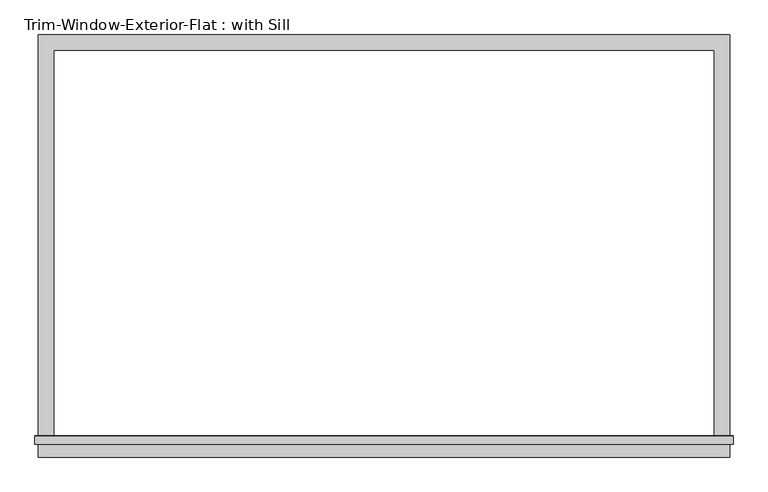
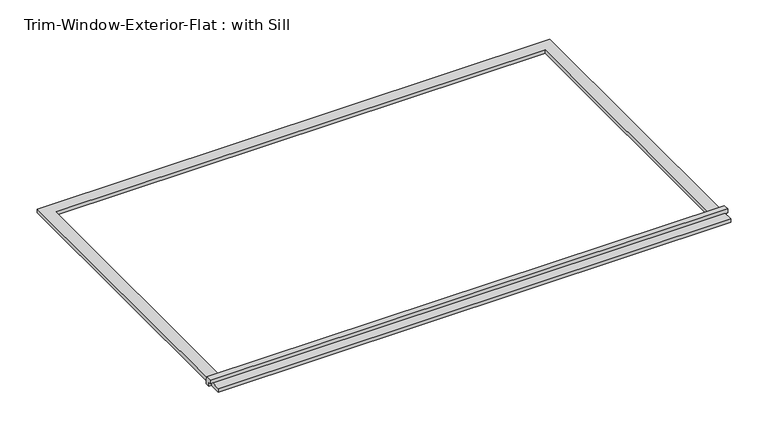
"""IFC4 building model written with IfcOpenShell, lengths in millimetres: proxy geometry, Trim-Window-Exterior-Flat : with Sill."""

from ifc_helpers import new_model, si_unit, frame, origin, origin_with_axes, place, context, project, spatial, polyline, outline, extrude, source, transform, mapped, element, save


def trim_window_exterior_flat_with_sill_cc36b48f(model_context):
    return source(origin(), model_context, "Body", "SweptSolid", [
        extrude(outline(polyline([(1276.35, -1444.5823709), (1276.35, -1501.7323709), (-1276.35, -1501.7323709), (-1276.35, -1444.5823709), (1276.35, -1444.5823709)])), origin_with_axes(), (0.0, 0.0, 1.0), 19.05),
        extrude(outline(polyline([(-1454.15, 38.1), (-1424.8580645, 38.1), (-1422.4, 19.05), (-1422.4, 0.0), (-1444.5823709, 0.0), (-1444.5823709, 19.05), (-1454.15, 19.05), (-1454.15, 38.1)])), frame((-1289.05, 0.0, 0.0), z_axis=(1.0, 0.0, 0.0), x_axis=(0.0, 1.0, 0.0)), (0.0, 0.0, 1.0), 2578.1),
        extrude(outline(polyline([(-1276.35, 57.15), (1276.35, 57.15), (1276.35, -1422.4), (1219.2, -1422.4), (1219.2, 0.0), (-1219.2, 0.0), (-1219.2, -1422.4), (-1276.35, -1422.4), (-1276.35, 57.15)])), origin_with_axes(), (0.0, 0.0, 1.0), 19.05),
    ])


if __name__ == "__main__":
    model = new_model("IFC4")
    model_context = context("Model", 3, world=origin())
    ifc_project = project(units=[si_unit("LENGTHUNIT", "METRE", prefix="MILLI")], contexts=[model_context])
    site = spatial("IfcSite", under=ifc_project)
    building = spatial("IfcBuilding", under=site)
    placement = place(None, origin())
    trim_window_exterior_flat_with_sill_shape = trim_window_exterior_flat_with_sill_cc36b48f(model_context)
    element("IfcBuildingElementProxy", 1, Name="Trim-Window-Exterior-Flat : with Sill", ObjectType="Trim-Window-Exterior-Flat : with Sill", at=placement, inside=building, context=model_context, shape_type="MappedRepresentation", body=[
        mapped(trim_window_exterior_flat_with_sill_shape, transform((0.0, 0.0, 0.0), x_axis=(1.0, 0.0, 0.0), y_axis=(0.0, 1.0, 0.0), z_axis=(0.0, 0.0, 1.0))),
    ])
    save(model, "model.ifc")

# Revit data of these elements
# Type "Trim-Window-Exterior-Flat : with Sill"
#   Trim Width = 0' - 2 1/4"
#   Trim Thickness_Picture Frame = 0' - 1 1/4"
#   Trim Thickness_with Sill = 0' - 0 3/4"
#   Sill Thickness = 0' - 1 1/4"
#   Opening Width [instance default] = 2' - 0"
#   Opening Height [instance default] = 3' - 0"
#   Default Elevation = 4' - 0"
#   Sill = yes
#   Picture Frame = no
#   Trim Material [instance default] = none
# Element 1 (IfcBuildingElementProxy, "Trim-Window-Exterior-Flat : with Sill")
#   Opening Width = 8' - 0"
#   Opening Height = 4' - 8"
#   Trim Material = Clad - White
#   Materials on its faces: "Clad - White"
# Materials
#   "Clad - White": class "Wood", colour RGB 245 245 243, transparency 0, Cost = 0
